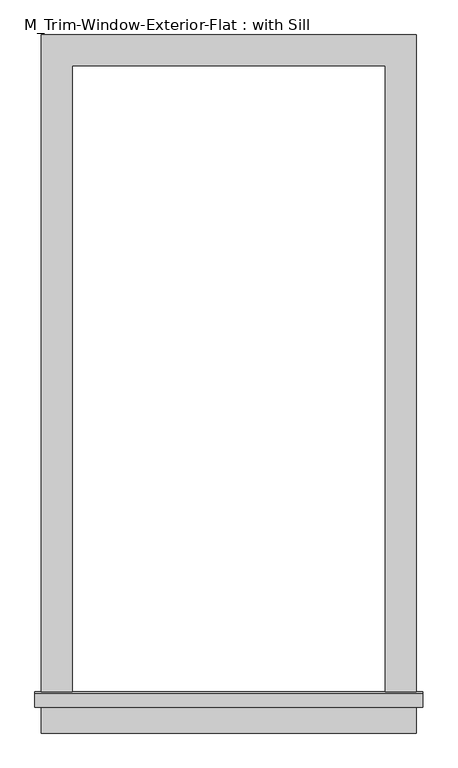
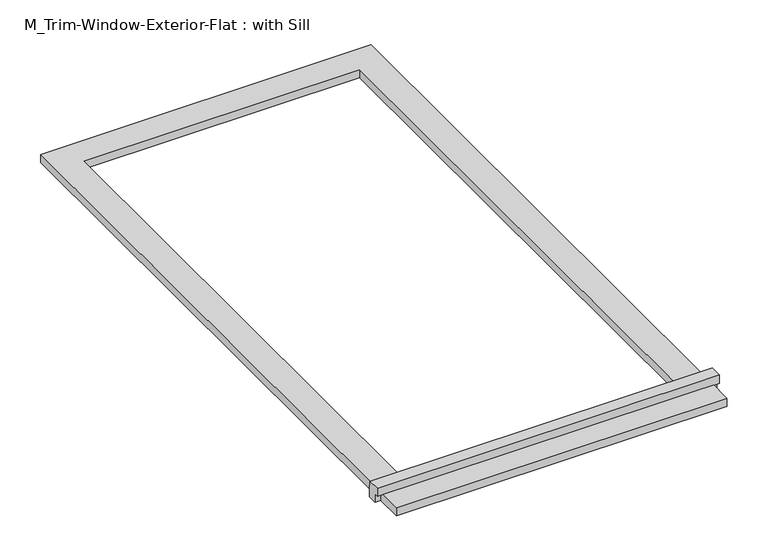
"""IFC4 building model written with IfcOpenShell, lengths in millimetres: proxy geometry, M_Trim-Window-Exterior-Flat : with Sill."""

from ifc_helpers import new_model, si_unit, frame, origin, origin_with_axes, place, context, project, spatial, polyline, outline, extrude, source, transform, mapped, element, save


def m_trim_window_exterior_flat_with_sill_2bc14f21(model_context):
    return source(origin(), model_context, "Body", "SweptSolid", [
        extrude(outline(polyline([(364.8, -1239.6323709), (364.8, -1299.6323709), (-364.8, -1299.6323709), (-364.8, -1239.6323709), (364.8, -1239.6323709)])), origin_with_axes(), (0.0, 0.0, 1.0), 19.05),
        extrude(outline(polyline([(-1249.2, 38.1), (-1221.6580645, 38.1), (-1219.2, 19.05), (-1219.2, 0.0), (-1239.6323709, 0.0), (-1239.6323709, 19.05), (-1249.2, 19.05), (-1249.2, 38.1)])), frame((-377.5, 0.0, 0.0), z_axis=(1.0, 0.0, 0.0), x_axis=(0.0, 1.0, 0.0)), (0.0, 0.0, 1.0), 755.0),
        extrude(outline(polyline([(-364.8, 60.0), (364.8, 60.0), (364.8, -1219.2), (304.8, -1219.2), (304.8, 0.0), (-304.8, 0.0), (-304.8, -1219.2), (-364.8, -1219.2), (-364.8, 60.0)])), origin_with_axes(), (0.0, 0.0, 1.0), 19.05),
    ])


if __name__ == "__main__":
    model = new_model("IFC4")
    model_context = context("Model", 3, world=origin())
    ifc_project = project(units=[si_unit("LENGTHUNIT", "METRE", prefix="MILLI")], contexts=[model_context])
    site = spatial("IfcSite", under=ifc_project)
    building = spatial("IfcBuilding", under=site)
    placement = place(None, origin())
    m_trim_window_exterior_flat_with_sill_shape = m_trim_window_exterior_flat_with_sill_2bc14f21(model_context)
    element("IfcBuildingElementProxy", 1, Name="M_Trim-Window-Exterior-Flat : with Sill", ObjectType="M_Trim-Window-Exterior-Flat : with Sill", at=placement, inside=building, context=model_context, shape_type="MappedRepresentation", body=[
        mapped(m_trim_window_exterior_flat_with_sill_shape, transform((0.0, 0.0, 0.0), x_axis=(1.0, 0.0, 0.0), y_axis=(0.0, 1.0, 0.0), z_axis=(0.0, 0.0, 1.0))),
    ])
    save(model, "model.ifc")

# Revit data of these elements
# Type "M_Trim-Window-Exterior-Flat : with Sill"
#   Trim Width = 0' - 2.3622"
#   Trim Thickness_Picture Frame = 0' - 1.1811"
#   Trim Thickness_with Sill = 0' - 0 3/4"
#   Sill Thickness = 0' - 1.1811"
#   Opening Width [instance default] = 1' - 11.62205"
#   Opening Height [instance default] = 2' - 11.43307"
#   Default Elevation = 3' - 11.24409"
#   Sill = yes
#   Picture Frame = no
#   Trim Material [instance default] = none
# Element 1 (IfcBuildingElementProxy, "M_Trim-Window-Exterior-Flat : with Sill")
#   Opening Width = 2' - 0"
#   Opening Height = 4' - 0"
#   Trim Material = Clad - White
#   Materials on its faces: "Clad - White"
# Materials
#   "Clad - White": class "Wood", colour RGB 242 242 238, transparency 0, Cost = 0
